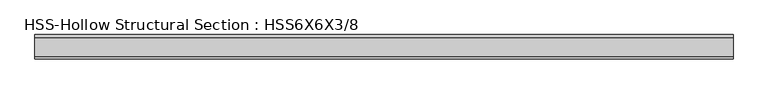
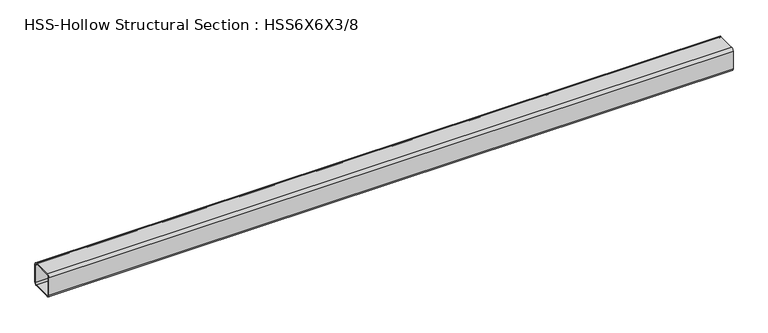
"""IFC4 building model written with IfcOpenShell, lengths in millimetres: member geometry, HSS-Hollow Structural Section : HSS6X6X3/8."""

from ifc_helpers import new_model, si_unit, point, frame, frame_2d, origin, place, context, project, spatial, polyline, circle_curve, trimmed, segment, composite_curve, outline, extrude, source, transform, mapped, element, save


def hss_hollow_structural_section_hss6x6x3_8_c14c5591(model_context):
    return source(origin(), model_context, "Body", "SweptSolid", [
        extrude(outline(composite_curve([segment(polyline([(76.2, 58.4708), (76.2, -58.4708)]), True, "CONTINUOUS"), segment(trimmed(circle_curve(frame_2d((58.4708, -58.4708)), 17.7292), [point((76.2, -58.4708))], [point((58.4708, -76.2))], False, "CARTESIAN"), True, "CONTINUOUS"), segment(polyline([(58.4708, -76.2), (-58.4708, -76.2)]), True, "CONTINUOUS"), segment(trimmed(circle_curve(frame_2d((-58.4708, -58.4708)), 17.7292), [point((-58.4708, -76.2))], [point((-76.2, -58.4708))], False, "CARTESIAN"), True, "CONTINUOUS"), segment(polyline([(-76.2, -58.4708), (-76.2, 58.4708)]), True, "CONTINUOUS"), segment(trimmed(circle_curve(frame_2d((-58.4708, 58.4708)), 17.7292), [point((-76.2, 58.4708))], [point((-58.4708, 76.2))], False, "CARTESIAN"), True, "CONTINUOUS"), segment(polyline([(-58.4708, 76.2), (58.4708, 76.2)]), True, "CONTINUOUS"), segment(trimmed(circle_curve(frame_2d((58.4708, 58.4708)), 17.7292), [point((58.4708, 76.2))], [point((76.2, 58.4708))], False, "CARTESIAN"), True, "CONTINUOUS")], self_intersect=False), holes=[composite_curve([segment(trimmed(circle_curve(frame_2d((-58.4708, 58.4708)), 8.8646), [point((-58.4708, 67.3354))], [point((-67.3354, 58.4708))], True, "CARTESIAN"), True, "CONTINUOUS"), segment(polyline([(-67.3354, 58.4708), (-67.3354, -58.4708)]), True, "CONTINUOUS"), segment(trimmed(circle_curve(frame_2d((-58.4708, -58.4708)), 8.8646), [point((-67.3354, -58.4708))], [point((-58.4708, -67.3354))], True, "CARTESIAN"), True, "CONTINUOUS"), segment(polyline([(-58.4708, -67.3354), (58.4708, -67.3354)]), True, "CONTINUOUS"), segment(trimmed(circle_curve(frame_2d((58.4708, -58.4708)), 8.8646), [point((58.4708, -67.3354))], [point((67.3354, -58.4708))], True, "CARTESIAN"), True, "CONTINUOUS"), segment(polyline([(67.3354, -58.4708), (67.3354, 58.4708)]), True, "CONTINUOUS"), segment(trimmed(circle_curve(frame_2d((58.4708, 58.4708)), 8.8646), [point((67.3354, 58.4708))], [point((58.4708, 67.3354))], True, "CARTESIAN"), True, "CONTINUOUS"), segment(polyline([(58.4708, 67.3354), (-58.4708, 67.3354)]), True, "CONTINUOUS")], self_intersect=False)]), frame((-2169.5251939, 0.0, 0.0), z_axis=(1.0, 0.0, 0.0), x_axis=(0.0, 1.0, 0.0)), (0.0, 0.0, 1.0), 4339.0503878),
    ])


if __name__ == "__main__":
    model = new_model("IFC4")
    model_context = context("Model", 3, world=origin())
    ifc_project = project(units=[si_unit("LENGTHUNIT", "METRE", prefix="MILLI")], contexts=[model_context])
    site = spatial("IfcSite", under=ifc_project)
    building = spatial("IfcBuilding", under=site)
    placement = place(None, origin())
    hss_hollow_structural_section_hss6x6x3_8_shape = hss_hollow_structural_section_hss6x6x3_8_c14c5591(model_context)
    element("IfcMember", 1, ObjectType="HSS-Hollow Structural Section : HSS6X6X3/8", at=placement, inside=building, context=model_context, shape_type="MappedRepresentation", body=[
        mapped(hss_hollow_structural_section_hss6x6x3_8_shape, transform((0.0, 0.0, 0.0), x_axis=(1.0, 0.0, 0.0), y_axis=(0.0, 1.0, 0.0), z_axis=(0.0, 0.0, 1.0))),
    ])
    save(model, "model.ifc")

# Revit data of these elements
# Type "HSS-Hollow Structural Section : HSS6X6X3/8"
#   Assembly Code = "B10"
#   Shape = "Square"
#   W = 27.4
#   Ht = 0' - 6"
#   Length [instance default] = 5' - 0"
#   b = 0' - 6"
#   kr = 0' - 0.698"
#   t = 0' - 0.349"
#   A = 0.0526389 SF
#   Structural Material [instance default] = Steel ASTM A500, Grade B, Rectangular and Square
# Element 1 (IfcMember, "HSS-Hollow Structural Section : HSS6X6X3/8")
#   Materials on its faces: "Steel ASTM A500, Grade B, Rectangular and Square"
# Materials
#   "Steel ASTM A500, Grade B, Rectangular and Square": class "Metal", colour RGB 199 199 199, transparency 0, Description = "Carbon steel", Cost = 0
